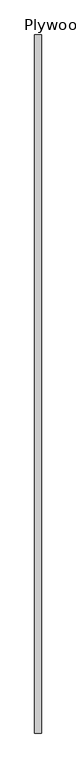
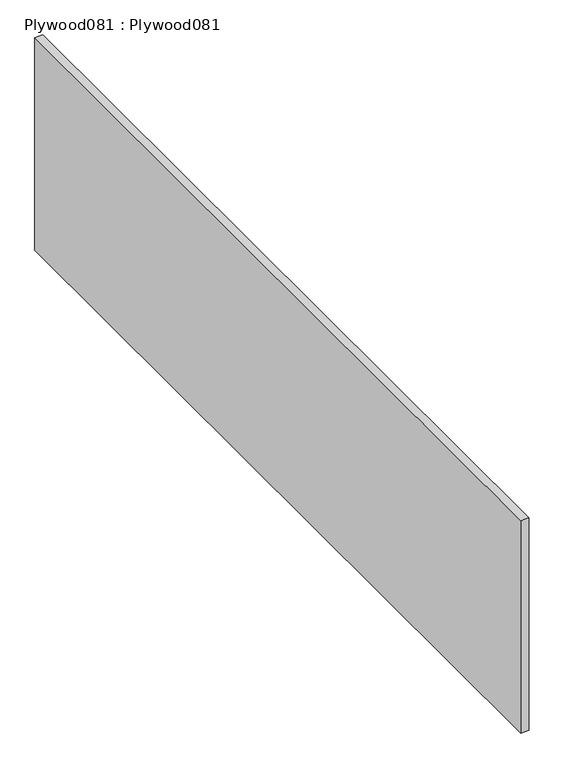
"""IFC4 building model written with IfcOpenShell, lengths in millimetres: proxy geometry, Plywood081 : Plywood081."""

from ifc_helpers import new_model, si_unit, frame, origin, place, context, project, spatial, polyline, outline, extrude, source, transform, mapped, element, save


def plywood081_plywood081_c43c3651(model_context):
    return source(origin(), model_context, "Body", "SweptSolid", [
        extrude(outline(polyline([(-2745.1737014, -1052.8906574), (-2764.2237014, -1052.8906574), (-2764.2237014, 947.1093426), (-2745.1737014, 947.1093426), (-2745.1737014, -1052.8906574)])), frame((0.0, 0.0, 39579.2960083), z_axis=(0.0, 0.0, 1.0), x_axis=(1.0, 0.0, 0.0)), (0.0, 0.0, 1.0), 533.3999917),
    ])


if __name__ == "__main__":
    model = new_model("IFC4")
    model_context = context("Model", 3, world=origin())
    ifc_project = project(units=[si_unit("LENGTHUNIT", "METRE", prefix="MILLI")], contexts=[model_context])
    site = spatial("IfcSite", under=ifc_project)
    building = spatial("IfcBuilding", under=site)
    placement = place(None, origin())
    plywood081_plywood081_shape = plywood081_plywood081_c43c3651(model_context)
    element("IfcBuildingElementProxy", 1, Name="Plywood081 : Plywood081", ObjectType="Plywood081 : Plywood081", at=placement, inside=building, context=model_context, shape_type="MappedRepresentation", body=[
        mapped(plywood081_plywood081_shape, transform((0.0, 0.0, 0.0), x_axis=(1.0, 0.0, 0.0), y_axis=(0.0, 1.0, 0.0), z_axis=(0.0, 0.0, 1.0))),
    ])
    save(model, "model.ifc")

# Revit data of these elements
# Type "Plywood081 : Plywood081"
#   NameOverride = "Plywood081"
# Element 1 (IfcBuildingElementProxy, "Plywood081 : Plywood081")
#   Materials on its faces: "CDX PLYWOOD -  SEE STRUCTURAL DWGS"
# Materials
#   "CDX PLYWOOD -  SEE STRUCTURAL DWGS": class "Unassigned", colour RGB 177 130 114, transparency 0, Cost = 0
